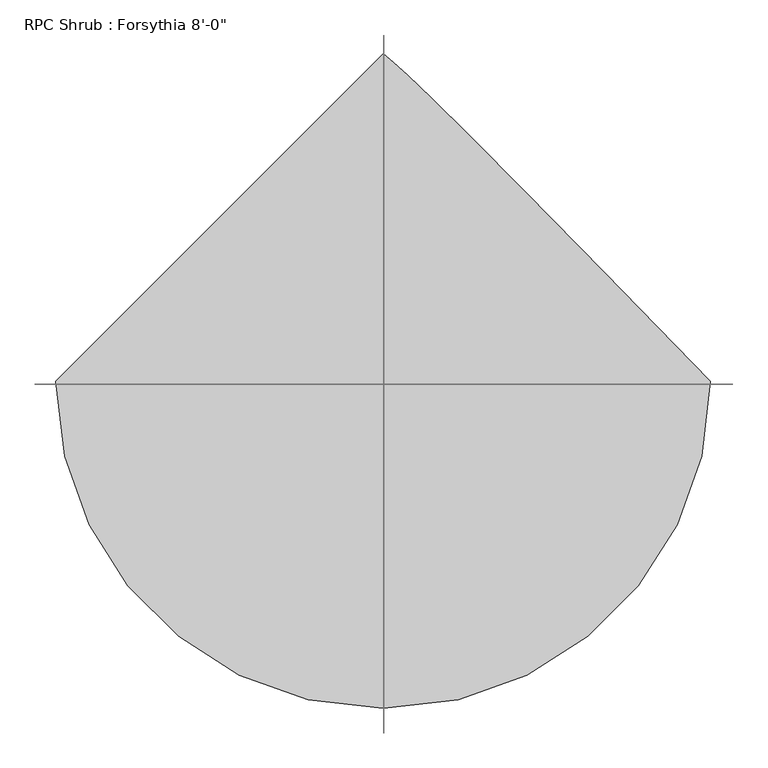
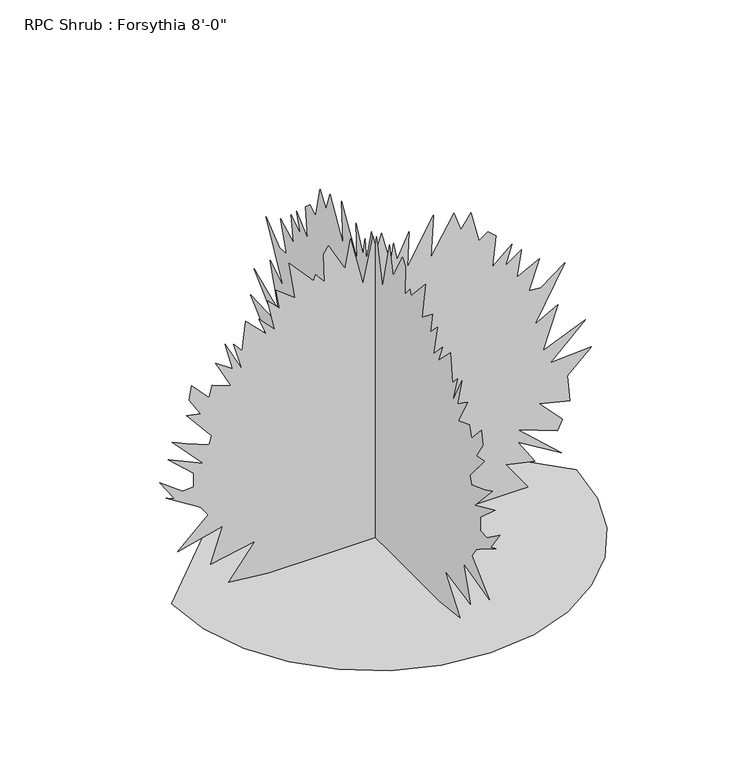
"""IFC4 building model written with IfcOpenShell, lengths in millimetres: geographic element geometry."""

from ifc_helpers import new_model, si_unit, origin, place, context, project, spatial, triangles, source, transform, mapped, element, save


def geographic_element_3ae10d36(model_context):
    return source(origin(), model_context, "Body", "Tessellation", [
        triangles([(-1519.5040535, 0.0, 0.0002833), (-1479.3336857, -348.1690825, 0.0002833), (-1364.9291862, -667.9078508, 0.0002833), (-1185.447191, -950.0545097, 0.0002833), (-950.0545097, -1185.447191, 0.0002833), (-667.9078508, -1364.9291862, 0.0002833), (-348.1690825, -1479.3336857, 0.0002833), (6.64e-05, -1519.5040535, 0.0002833), (348.1690825, -1479.3336857, 0.0002833), (667.9078508, -1364.9291862, 0.0002833), (950.0545097, -1185.447191, 0.0002833), (1185.447191, -950.0545097, 0.0002833), (1364.9291862, -667.9078508, 0.0002833), (1479.3336857, -348.1690825, 0.0002833), (1519.5040535, 0.0001328, 0.0002833), (1025.698439, 506.5233338, 0.0002833), (659.6172232, 879.4549673, 0.0002833), (399.9699903, 1141.05804, 0.0002833), (225.4722113, 1313.5981625, 0.0002833), (114.8360501, 1419.3438881, 0.0002833), (46.774248, 1480.5555588, 0.0002833), (-0.0001993, 1519.5040535, 0.0002833), (-792.3428427, -13.4822871, 0.037948), (-1099.2418425, -13.4822621, 31.9687972), (-901.0348274, -13.4822871, 287.7194292), (-1233.5117718, -13.4822871, 223.7813261), (-1143.9993576, -13.4822871, 492.3196223), (-1482.8669003, -13.4822871, 409.2003862), (-1252.691415, -13.482312, 620.1937574), (-1310.2352863, -13.482312, 703.3130299), (-1565.9861, -13.482312, 863.1557442), (-1502.0490143, -13.482312, 837.5804157), (-1617.1342861, -13.482312, 1003.8188152), (-1444.505143, -13.482312, 875.9446438), (-1361.3859432, -13.482312, 882.3378582), (-1361.3859432, -13.482312, 991.0299156), (-1553.1972004, -13.4823382, 1163.6615295), (-1291.0531723, -13.4823382, 1042.1805725), (-1521.2286575, -13.4823382, 1291.5383171), (-1412.5366001, -13.4823382, 1240.3875149), (-1246.2982006, -13.4823382, 1176.4505018), (-1227.1160866, -13.4823382, 1240.3875149), (-1412.5366001, -13.4823382, 1464.1673149), (-1310.2352863, -13.4823382, 1444.987817), (-1393.3544861, -13.4823631, 1579.2552029), (-1374.1723721, -13.4823631, 1687.9497311), (-1246.2982006, -13.4823631, 1547.28666), (-1220.7228722, -13.4823631, 1636.7990742), (-1080.0597284, -13.4823631, 1585.6482719), (-1195.147471, -13.4823631, 1803.0374737), (-1067.2732996, -13.4823631, 1713.5250595), (-1124.8171709, -13.4823881, 1930.9116451), (-996.9429995, -13.4823631, 1687.9497311), (-1060.8800852, -13.4823881, 1905.3363167), (-996.9429995, -13.4823631, 1835.0060165), (-971.367671, -13.4823881, 2058.7858166), (-817.9181711, -13.4823881, 1905.3363167), (-869.0663572, -13.4823881, 2039.6061733), (-753.9785419, -13.4823881, 1918.1252163), (-805.1292715, -13.4823881, 2161.0871304), (-715.6167847, -13.4823881, 2071.5747162), (-741.1921858, -13.4823881, 2225.0242161), (-600.5290421, -13.4823881, 2116.3296879), (-645.2865572, -13.4824142, 2404.0490444), (-459.8659347, -13.4823881, 2199.4488876), (-447.0795422, -13.4823881, 2244.2063301), (-379.2689283, -13.4823881, 2162.8804802), (-385.6646862, -13.4824142, 2386.6602802), (-347.290248, -13.4824142, 2438.4078484), (-223.176294, -13.4824142, 2213.9981449), (-182.9654127, -13.4823631, 2435.1743248), (-90.8322191, -13.4823631, 2047.6376598), (-12.3045871, -13.4824142, 2397.6559753), (13.2704245, -13.4823881, 2276.174873), (51.6330312, -13.4824142, 2397.6559753), (115.5706256, -13.4823881, 2135.5118019), (141.1454544, -13.4823881, 2288.9613018), (166.7205467, -13.4823881, 2148.2982307), (256.2334877, -13.4824142, 2340.1119587), (243.445551, -13.4823881, 2065.1815018), (441.6515305, -13.4824142, 2404.0490444), (422.4693801, -13.4823881, 2077.9679306), (595.1010303, -13.4824142, 2365.6874325), (646.2517599, -13.4823881, 2218.6310017), (722.9777452, -13.4824142, 2327.3230591), (780.5216166, -13.4823881, 2084.361145), (850.8519167, -13.4823881, 2129.1185875), (908.395788, -13.4823881, 2077.9679306), (882.8204596, -13.4823631, 1841.399231), (1029.876745, -13.4823881, 1969.2734024), (978.7260881, -13.4823631, 1815.8239025), (1100.2070452, -13.4823881, 1898.9431023), (1068.2385023, -13.4823631, 1694.3429455), (1234.4769745, -13.4823631, 1783.8553596), (1157.7509165, -13.4823631, 1553.6797291), (1247.2634033, -13.4823631, 1547.28666), (1426.2882317, -13.4823631, 1681.5565166), (1202.5084316, -13.4823382, 1272.3560577), (1375.1400455, -13.4823382, 1368.2616863), (1260.0523029, -13.4823382, 1042.1805725), (1579.7377316, -13.4823382, 1176.4505018), (1317.5961742, -13.482312, 927.0928299), (1624.495174, -13.482312, 946.2749439), (1445.4703457, -13.482312, 780.0364717), (1464.6524597, -13.4822871, 575.436315), (1234.4769745, -13.482312, 632.9801863), (1407.1085884, -13.4822871, 447.5621435), (1368.7443604, -13.4822871, 370.838629), (1074.6317167, -13.4822871, 479.5306864), (1400.7129032, -13.4822871, 185.418824), (1074.6317167, -13.4822871, 383.6250578), (1202.5084316, -13.4822871, 185.418824), (985.1193026, -13.4822871, 236.568736), (1151.4898161, -13.4822871, 0.0386752), (19.664159, -13.4822621, 0.0001234), (3.6800653, -809.5031324, 0.0378489), (3.68004, -1116.4046757, 31.9687972), (3.6800653, -918.1977333, 287.7194292), (3.6800653, -1250.6720615, 223.7813261), (3.6800653, -1161.1596474, 492.3196223), (3.6800653, -1500.0298061, 409.2003862), (3.6800653, -1269.8541756, 620.1937574), (3.6800653, -1327.3980469, 703.3130299), (3.6800908, -1583.1463898, 863.1557442), (3.6800908, -1519.209304, 837.5804157), (3.6800908, -1634.2970467, 1003.8188152), (3.6800908, -1461.6654327, 875.9446438), (3.6800908, -1378.5487038, 882.3378582), (3.6800908, -1378.5487038, 991.0299156), (3.6800908, -1570.3599609, 1163.6615295), (3.6800908, -1308.2159328, 1042.1805725), (3.6800908, -1538.3914181, 1291.5383171), (3.6800908, -1429.6968899, 1240.3875149), (3.6800908, -1263.4609612, 1176.4505018), (3.6800908, -1244.2788471, 1240.3875149), (3.6800908, -1429.6968899, 1464.1673149), (3.6800908, -1327.3980469, 1444.987817), (3.6800908, -1410.5172466, 1579.2552029), (3.6801161, -1391.3351326, 1687.9497311), (3.6800908, -1263.4609612, 1547.28666), (3.6800908, -1237.8856327, 1636.7990742), (3.6800908, -1097.2225616, 1585.6508881), (3.6801161, -1212.3103043, 1803.0374737), (3.6800908, -1084.4361328, 1713.5250595), (3.6801161, -1141.9800041, 1930.9116451), (3.6800908, -1014.1032892, 1687.9497311), (3.6801161, -1078.0403749, 1905.3363167), (3.6800908, -1014.1032892, 1835.0060165), (3.6801161, -988.5305042, 2058.7858166), (3.6800908, -835.0784609, 1905.3363167), (3.6801161, -886.2291904, 2039.6061733), (3.6800908, -771.1413752, 1918.1252163), (3.6801161, -822.2921047, 2161.0871304), (3.6801161, -732.7796179, 2071.5747162), (3.6801161, -758.355019, 2225.0242161), (3.6801161, -617.6918753, 2116.3296879), (3.6801161, -662.446847, 2404.0490444), (3.6801161, -477.0287679, 2199.4488876), (3.6801161, -464.2423754, 2244.2063301), (3.6801161, -396.4317616, 2162.8804802), (3.6801161, -402.824976, 2386.6602802), (3.6801161, -364.4530812, 2438.4078484), (3.6801161, -240.3386185, 2213.9981449), (3.6800653, -200.1277554, 2435.1743248), (3.6800653, -107.994798, 2047.640276), (3.6801161, -29.4668878, 2397.6559753), (3.6800908, -3.8919275, 2276.174873), (3.6801161, 34.4707044, 2397.6559753), (3.6800908, 98.408301, 2135.5118019), (3.6800908, 123.9831299, 2288.9613018), (3.6800908, 149.5579678, 2148.3008469), (3.6800908, 239.0706363, 2340.1119587), (3.6800908, 226.2832264, 2065.1815018), (3.6800908, 424.4886972, 2404.0490444), (3.6800908, 405.3090903, 2077.9679306), (3.6800908, 577.9381971, 2365.6874325), (3.6800908, 629.0889267, 2218.6310017), (3.6800908, 705.814912, 2327.3256752), (3.6800908, 763.3587833, 2084.361145), (3.6800908, 833.6890835, 2129.1185875), (3.6800908, 891.2329548, 2077.9679306), (3.6800653, 865.6576263, 1841.399231), (3.6800653, 1012.7139118, 1969.2734024), (3.6800653, 961.5632549, 1815.8239025), (3.6800653, 1083.044212, 1898.9431023), (3.6800653, 1051.0756691, 1694.3429455), (3.6800653, 1217.3141413, 1783.8553596), (3.6800653, 1140.5880833, 1553.6797291), (3.6800653, 1230.1004974, 1547.28666), (3.6800653, 1409.1253258, 1681.5565166), (3.6800653, 1185.3455984, 1272.3560577), (3.6800653, 1357.977285, 1368.2616863), (3.68004, 1242.8895424, 1042.1805725), (3.68004, 1562.5774418, 1176.4505018), (3.68004, 1300.4334137, 927.0928299), (3.68004, 1607.3324135, 946.2749439), (3.68004, 1428.3075851, 780.0364717), (3.68004, 1447.4896992, 575.436315), (3.68004, 1217.3141413, 632.9801863), (3.6800145, 1389.9458279, 447.5621435), (3.6800145, 1351.5840706, 370.838629), (3.68004, 1057.471427, 479.5306864), (3.6800145, 1383.5526134, 185.4185696), (3.68004, 1057.471427, 383.6250578), (3.6800145, 1185.3455984, 185.4185696), (3.6800145, 967.9590128, 236.568736), (3.68004, 1134.3269829, 0.038518), (3.68004, 2.5017556, 0.0)], [[21, 22, 1], [20, 21, 1], [19, 20, 1], [18, 19, 1], [17, 18, 1], [17, 1, 2], [17, 2, 3], [17, 3, 4], [16, 17, 4], [16, 4, 5], [16, 5, 6], [16, 6, 7], [16, 7, 8], [16, 8, 9], [16, 9, 10], [16, 10, 11], [16, 11, 12], [15, 16, 12], [14, 15, 12], [13, 14, 12], [30, 31, 32], [109, 110, 111], [51, 52, 53], [36, 37, 38], [32, 33, 34], [76, 77, 78], [100, 101, 102], [38, 39, 40], [78, 79, 80], [57, 58, 59], [70, 71, 72], [96, 97, 98], [72, 73, 74], [53, 54, 55], [80, 81, 82], [49, 50, 51], [27, 28, 29], [89, 90, 91], [74, 75, 76], [59, 60, 61], [63, 64, 65], [38, 40, 41], [102, 103, 104], [42, 43, 44], [98, 99, 100], [61, 62, 63], [93, 94, 95], [111, 112, 113], [91, 92, 93], [84, 85, 86], [82, 83, 84], [55, 56, 57], [45, 46, 47], [44, 45, 47], [113, 114, 115], [65, 66, 67], [23, 24, 25], [72, 74, 76], [25, 26, 27], [68, 69, 70], [67, 68, 70], [30, 32, 34], [30, 34, 35], [104, 105, 106], [49, 51, 53], [102, 104, 106], [95, 96, 98], [47, 48, 49], [107, 108, 109], [106, 107, 109], [82, 84, 86], [86, 87, 88], [86, 88, 89], [67, 70, 72], [115, 23, 25], [53, 55, 57], [82, 86, 89], [76, 78, 80], [63, 65, 67], [59, 61, 63], [42, 44, 47], [42, 47, 49], [35, 36, 38], [72, 76, 80], [111, 113, 115], [109, 111, 115], [100, 102, 106], [100, 106, 109], [100, 109, 115], [98, 100, 115], [98, 115, 25], [95, 98, 25], [93, 95, 25], [91, 93, 25], [89, 91, 25], [82, 89, 25], [80, 82, 25], [72, 80, 25], [72, 25, 27], [72, 27, 29], [67, 72, 29], [63, 67, 29], [59, 63, 29], [59, 29, 30], [59, 30, 35], [59, 35, 38], [59, 38, 41], [59, 41, 42], [59, 42, 49], [59, 49, 53], [59, 53, 57], [123, 124, 125], [202, 203, 204], [144, 145, 146], [129, 130, 131], [125, 126, 127], [169, 170, 171], [193, 194, 195], [131, 132, 133], [171, 172, 173], [150, 151, 152], [163, 164, 165], [189, 190, 191], [165, 166, 167], [146, 147, 148], [173, 174, 175], [142, 143, 144], [120, 121, 122], [182, 183, 184], [167, 168, 169], [152, 153, 154], [156, 157, 158], [131, 133, 134], [195, 196, 197], [135, 136, 137], [191, 192, 193], [154, 155, 156], [186, 187, 188], [204, 205, 206], [184, 185, 186], [177, 178, 179], [175, 176, 177], [148, 149, 150], [138, 139, 140], [137, 138, 140], [206, 207, 208], [158, 159, 160], [116, 117, 118], [165, 167, 169], [118, 119, 120], [161, 162, 163], [160, 161, 163], [123, 125, 127], [123, 127, 128], [197, 198, 199], [142, 144, 146], [195, 197, 199], [188, 189, 191], [140, 141, 142], [200, 201, 202], [199, 200, 202], [175, 177, 179], [179, 180, 181], [179, 181, 182], [160, 163, 165], [208, 116, 118], [146, 148, 150], [175, 179, 182], [169, 171, 173], [156, 158, 160], [152, 154, 156], [135, 137, 140], [135, 140, 142], [128, 129, 131], [165, 169, 173], [204, 206, 208], [202, 204, 208], [193, 195, 199], [193, 199, 202], [193, 202, 208], [191, 193, 208], [191, 208, 118], [188, 191, 118], [186, 188, 118], [184, 186, 118], [182, 184, 118], [175, 182, 118], [173, 175, 118], [165, 173, 118], [165, 118, 120], [165, 120, 122], [160, 165, 122], [156, 160, 122], [152, 156, 122], [152, 122, 123], [152, 123, 128], [152, 128, 131], [152, 131, 134], [152, 134, 135], [152, 135, 142], [152, 142, 146], [152, 146, 150]], closed=False),
    ])


if __name__ == "__main__":
    model = new_model("IFC4")
    model_context = context("Model", 3, world=origin())
    ifc_project = project(units=[si_unit("LENGTHUNIT", "METRE", prefix="MILLI")], contexts=[model_context])
    site = spatial("IfcSite", under=ifc_project)
    building = spatial("IfcBuilding", under=site)
    placement = place(None, origin())
    geographic_element_shape = geographic_element_3ae10d36(model_context)
    element("IfcGeographicElement", 1, ObjectType="RPC Shrub : Forsythia 8'-0\"", at=placement, inside=building, context=model_context, shape_type="MappedRepresentation", body=[
        mapped(geographic_element_shape, transform((0.0, 0.0, 0.0), x_axis=(1.0, 0.0, 0.0), y_axis=(0.0, 1.0, 0.0), z_axis=(0.0, 0.0, 1.0))),
    ])
    save(model, "model.ifc")

# Revit data of these elements
# Type "RPC Shrub : Forsythia 8'-0\""
#   Type Comments = "Forsythia"
#   built-in parameter 1005198 = "{2, 15},{39, RPC-16-G2F6-877X-GLVN-N000-ST1L-LVER-AU},{1, 0},{1, 0},{2, 13},{1, 8},{5, Color},{1, 0},{1, 0},{3, 0.8},{3, 0.8},{3, 0.8},{1, 8},{7, BBoxMin},{1, 0},{1, 0},{1, 0},{1, 0},{1, 0},{1, 8},{7, BBoxMax},{1, 0},{1, 0},{1, 0},{1, 0},{1, 0},{2, 11},{9, RPCTypeId},{1, 0},{1, 0},{39, RPC-16-G2F6-877X-GLVN-N000-ST1L-LVER-AU},{1, 6},{14, RPCPlantHeight},{1, 0},{1, 0},{1, 8},{2, 11},{7, keyword},{1, 0},{1, 0},{35, :RPCs:Shrubs & Grasses:Geometry:RPC},{2, 11},{8, category},{1, 0},{1, 0},{16, Shrubs & Grasses},{2, 11},{12, LocalizedUID},{1, 0},{1, 0},{9, Forsythia},{2, 14},{6, Height},{1, 0},{1, 0},{1, 8},{1, 2},{16, Cast Reflections},{1, 0},{1, 0},{1, 0},{1, 2},{12, Cast Shadows},{1, 0},{1, 0},{1, 1},{1, 2},{9, Lock View},{1, 0},{1, 0},{1, 0},{1, 4},{5, ViewC},{1, 0},{1, 0},{1, 0},{21, assetlibrary_base.fbx},{1, 5},"
#   built-in parameter 1005195 = "RPC-16-G2F6-877X-GLVN-N000-ST1L-LVER-AU"
#   Assembly Code = "G2050500"
#   Height = 8' - 0"
